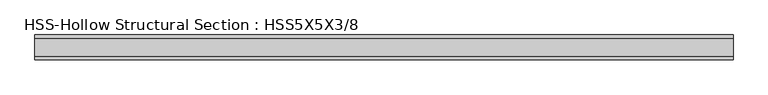
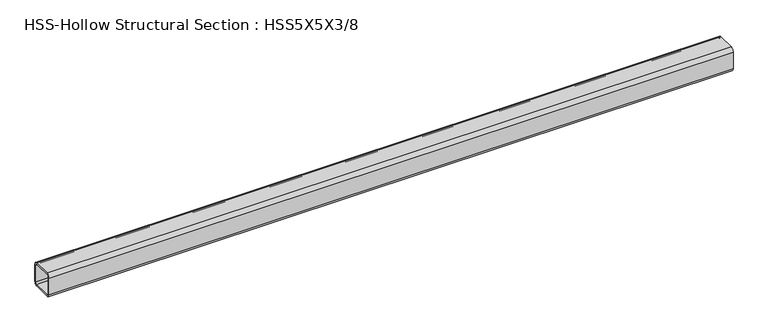
"""IFC4 building model written with IfcOpenShell, lengths in millimetres: member geometry, HSS-Hollow Structural Section : HSS5X5X3/8."""

from ifc_helpers import new_model, si_unit, point, frame, frame_2d, origin, place, context, project, spatial, polyline, circle_curve, trimmed, segment, composite_curve, outline, extrude, source, transform, mapped, element, save


def hss_hollow_structural_section_hss5x5x3_8_63cfa585(model_context):
    return source(origin(), model_context, "Body", "SweptSolid", [
        extrude(outline(composite_curve([segment(polyline([(63.5, 45.7708), (63.5, -45.7708)]), True, "CONTINUOUS"), segment(trimmed(circle_curve(frame_2d((45.7708, -45.7708)), 17.7292), [point((63.5, -45.7708))], [point((45.7708, -63.5))], False, "CARTESIAN"), True, "CONTINUOUS"), segment(polyline([(45.7708, -63.5), (-45.7708, -63.5)]), True, "CONTINUOUS"), segment(trimmed(circle_curve(frame_2d((-45.7708, -45.7708)), 17.7292), [point((-45.7708, -63.5))], [point((-63.5, -45.7708))], False, "CARTESIAN"), True, "CONTINUOUS"), segment(polyline([(-63.5, -45.7708), (-63.5, 45.7708)]), True, "CONTINUOUS"), segment(trimmed(circle_curve(frame_2d((-45.7708, 45.7708)), 17.7292), [point((-63.5, 45.7708))], [point((-45.7708, 63.5))], False, "CARTESIAN"), True, "CONTINUOUS"), segment(polyline([(-45.7708, 63.5), (45.7708, 63.5)]), True, "CONTINUOUS"), segment(trimmed(circle_curve(frame_2d((45.7708, 45.7708)), 17.7292), [point((45.7708, 63.5))], [point((63.5, 45.7708))], False, "CARTESIAN"), True, "CONTINUOUS")], self_intersect=False), holes=[composite_curve([segment(trimmed(circle_curve(frame_2d((-45.7708, 45.7708)), 8.8646), [point((-45.7708, 54.6354))], [point((-54.6354, 45.7708))], True, "CARTESIAN"), True, "CONTINUOUS"), segment(polyline([(-54.6354, 45.7708), (-54.6354, -45.7708)]), True, "CONTINUOUS"), segment(trimmed(circle_curve(frame_2d((-45.7708, -45.7708)), 8.8646), [point((-54.6354, -45.7708))], [point((-45.7708, -54.6354))], True, "CARTESIAN"), True, "CONTINUOUS"), segment(polyline([(-45.7708, -54.6354), (45.7708, -54.6354)]), True, "CONTINUOUS"), segment(trimmed(circle_curve(frame_2d((45.7708, -45.7708)), 8.8646), [point((45.7708, -54.6354))], [point((54.6354, -45.7708))], True, "CARTESIAN"), True, "CONTINUOUS"), segment(polyline([(54.6354, -45.7708), (54.6354, 45.7708)]), True, "CONTINUOUS"), segment(trimmed(circle_curve(frame_2d((45.7708, 45.7708)), 8.8646), [point((54.6354, 45.7708))], [point((45.7708, 54.6354))], True, "CARTESIAN"), True, "CONTINUOUS"), segment(polyline([(45.7708, 54.6354), (-45.7708, 54.6354)]), True, "CONTINUOUS")], self_intersect=False)]), frame((-1783.4477506, 0.0, 0.0), z_axis=(1.0, 0.0, 0.0), x_axis=(0.0, 1.0, 0.0)), (0.0, 0.0, 1.0), 3566.8955011),
    ])


if __name__ == "__main__":
    model = new_model("IFC4")
    model_context = context("Model", 3, world=origin())
    ifc_project = project(units=[si_unit("LENGTHUNIT", "METRE", prefix="MILLI")], contexts=[model_context])
    site = spatial("IfcSite", under=ifc_project)
    building = spatial("IfcBuilding", under=site)
    placement = place(None, origin())
    hss_hollow_structural_section_hss5x5x3_8_shape = hss_hollow_structural_section_hss5x5x3_8_63cfa585(model_context)
    element("IfcMember", 1, ObjectType="HSS-Hollow Structural Section : HSS5X5X3/8", at=placement, inside=building, context=model_context, shape_type="MappedRepresentation", body=[
        mapped(hss_hollow_structural_section_hss5x5x3_8_shape, transform((0.0, 0.0, 0.0), x_axis=(1.0, 0.0, 0.0), y_axis=(0.0, 1.0, 0.0), z_axis=(0.0, 0.0, 1.0))),
    ])
    save(model, "model.ifc")

# Revit data of these elements
# Type "HSS-Hollow Structural Section : HSS5X5X3/8"
#   Assembly Code = "B10"
#   Shape = "Square"
#   W = 22.3
#   Ht = 0' - 5"
#   Length [instance default] = 5' - 0"
#   b = 0' - 5"
#   kr = 0' - 0.698"
#   t = 0' - 0.349"
#   A = 0.0429167 SF
#   Structural Material [instance default] = Steel ASTM A500, Grade B, Rectangular and Square
# Element 1 (IfcMember, "HSS-Hollow Structural Section : HSS5X5X3/8")
#   Materials on its faces: "Steel ASTM A500, Grade B, Rectangular and Square"
# Materials
#   "Steel ASTM A500, Grade B, Rectangular and Square": class "Metal", colour RGB 199 199 199, transparency 0, Description = "Carbon steel", Cost = 0
